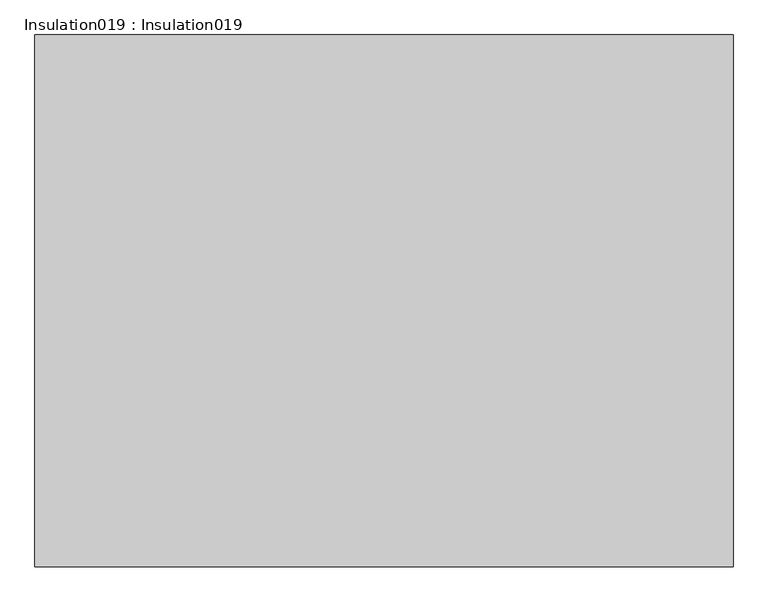
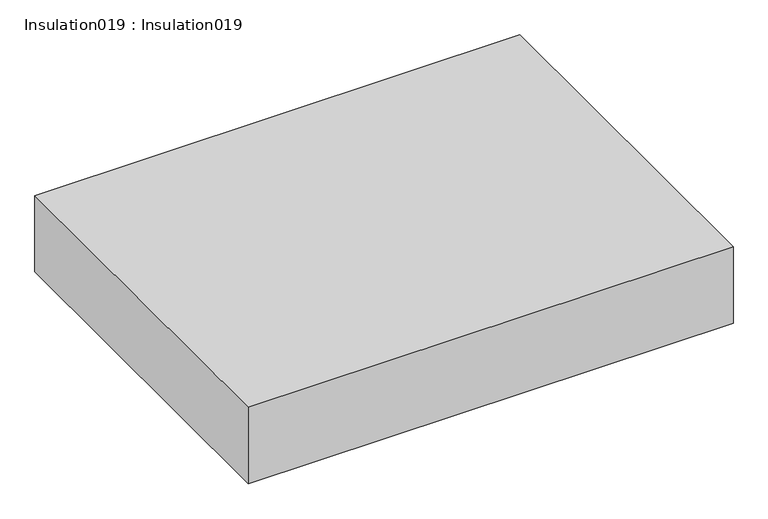
"""IFC4 building model written with IfcOpenShell, lengths in millimetres: proxy geometry, Insulation019 : Insulation019."""

import ifcopenshell
import ifcopenshell.guid

model = None  # the IFC model being written
_history = None  # IfcOwnerHistory: only IFC2X3 demands one
_inside = {}  # id of a spatial element -> (the spatial element, [elements in it])
_under = {}  # id of a project, library or spatial element -> (it, [spatial elements below it])
_declared = {}  # id of a project -> (the project, [libraries it declares])
_typed = {}  # id of a type object -> (the type object, [elements of that type])
_made_of = {}  # id of a material, layer set ... -> (it, [elements and type objects made of it])


def new_model(schema):
    """Start an empty IFC model of exactly this schema.

    Asked for "IFC4X3", IfcOpenShell would pick the latest addendum, in which some entities
    have other attributes; the version numbers below select the first issue.
    IFC2X3 requires an IfcOwnerHistory on every rooted entity: one is made here for all.
    """
    global model, _history
    if schema == "IFC4X3":
        model = ifcopenshell.file(schema_version=(4, 3, 0, 0))
    else:
        model = ifcopenshell.file(schema=schema)
    _inside.clear()
    _under.clear()
    _declared.clear()
    _typed.clear()
    _made_of.clear()
    _history = None
    if model.schema == "IFC2X3":
        org = make("IfcOrganization", Name="unknown")
        user = make(
            "IfcPersonAndOrganization",
            ThePerson=make("IfcPerson", FamilyName="unknown"),
            TheOrganization=org,
        )
        app = make(
            "IfcApplication",
            ApplicationDeveloper=org,
            Version="unknown",
            ApplicationFullName="unknown",
            ApplicationIdentifier="unknown",
        )
        _history = make(
            "IfcOwnerHistory",
            OwningUser=user,
            OwningApplication=app,
            ChangeAction="ADDED",
            CreationDate=0,
        )
    return model


def make(cls, **values):
    """One entity of the class cls with the attributes given. An attribute that is None is left unset."""
    return model.create_entity(
        cls, **{name: value for name, value in values.items() if value is not None}
    )


def rooted(cls, **values):
    """An entity with a GlobalId (a new one), such as an element, a storey or a relation."""
    return make(cls, GlobalId=ifcopenshell.guid.new(), OwnerHistory=_history, **values)


def si_unit(unit_type, name, prefix=None):
    """IfcSIUnit, for example si_unit("LENGTHUNIT", "METRE", prefix="MILLI")."""
    return make("IfcSIUnit", UnitType=unit_type, Prefix=prefix, Name=name)


def assignment(units):
    """IfcUnitAssignment: the units of a project."""
    return None if units is None else make("IfcUnitAssignment", Units=units)


def point(xyz):
    """IfcCartesianPoint."""
    return None if xyz is None else make("IfcCartesianPoint", Coordinates=xyz)


def direction(xyz):
    """IfcDirection."""
    return None if xyz is None else make("IfcDirection", DirectionRatios=xyz)


def frame(location, z_axis=None, x_axis=None):
    """IfcAxis2Placement3D, a coordinate frame: its origin and axes. An axis left out is left unset."""
    return make(
        "IfcAxis2Placement3D",
        Location=point(location),
        Axis=direction(z_axis),
        RefDirection=direction(x_axis),
    )


def origin():
    """The frame at (0, 0, 0) with its axes left unset."""
    return frame((0.0, 0.0, 0.0))


def place(relative_to, where):
    """IfcLocalPlacement: puts the frame where relative to a parent placement (None: the world)."""
    return make(
        "IfcLocalPlacement", PlacementRelTo=relative_to, RelativePlacement=where
    )


def context(
    kind, dimensions, precision=None, world=None, true_north=None, identifier=None
):
    """IfcGeometricRepresentationContext, for example the 3D "Model" context."""
    return make(
        "IfcGeometricRepresentationContext",
        ContextIdentifier=identifier,
        ContextType=kind,
        CoordinateSpaceDimension=dimensions,
        Precision=precision,
        WorldCoordinateSystem=world,
        TrueNorth=true_north,
    )


def project(units=None, contexts=None):
    """IfcProject with its units and contexts."""
    return rooted(
        "IfcProject",
        Name="project",
        RepresentationContexts=contexts,
        UnitsInContext=assignment(units),
    )


def spatial(cls, under=None, at=None, **own):
    """A site, building, storey or space (cls), placed at a placement, below another one or the project."""
    s = rooted(cls, ObjectPlacement=at, **own)
    if under is not None:
        _under.setdefault(under.id(), (under, []))[1].append(s)
    return s


def polyline(points):
    """IfcPolyline through the points."""
    return make("IfcPolyline", Points=[point(p) for p in points])


def outline(outer, holes=None, kind="AREA"):
    """IfcArbitraryClosedProfileDef: a profile drawn as a closed curve; with holes, ...WithVoids."""
    if holes is None:
        return make("IfcArbitraryClosedProfileDef", ProfileType=kind, OuterCurve=outer)
    return make(
        "IfcArbitraryProfileDefWithVoids",
        ProfileType=kind,
        OuterCurve=outer,
        InnerCurves=holes,
    )


def extrude(swept, where, along, depth):
    """IfcExtrudedAreaSolid: the profile swept, set in the frame where, extruded along a direction by depth."""
    return make(
        "IfcExtrudedAreaSolid",
        SweptArea=swept,
        Position=where,
        ExtrudedDirection=direction(along),
        Depth=depth,
    )


def shape(context_of_items, identifier, shape_type, items):
    """IfcShapeRepresentation: the items that make up one representation, for example the "Body"."""
    return make(
        "IfcShapeRepresentation",
        ContextOfItems=context_of_items,
        RepresentationIdentifier=identifier,
        RepresentationType=shape_type,
        Items=items,
    )


def source(mapping_origin, context_of_items, identifier, shape_type, items):
    """IfcRepresentationMap: a shape defined once, which mapped items show again and again."""
    return make(
        "IfcRepresentationMap",
        MappingOrigin=mapping_origin,
        MappedRepresentation=shape(context_of_items, identifier, shape_type, items),
    )


def transform(
    local_origin,
    x_axis=None,
    y_axis=None,
    z_axis=None,
    scale=None,
    scale2=None,
    scale3=None,
    uniform=True,
):
    """IfcCartesianTransformationOperator3D, or its non-uniform kind. x_axis, y_axis, z_axis: its Axis1, 2, 3."""
    if uniform:
        return make(
            "IfcCartesianTransformationOperator3D",
            Axis1=direction(x_axis),
            Axis2=direction(y_axis),
            LocalOrigin=point(local_origin),
            Scale=scale,
            Axis3=direction(z_axis),
        )
    return make(
        "IfcCartesianTransformationOperator3DnonUniform",
        Axis1=direction(x_axis),
        Axis2=direction(y_axis),
        LocalOrigin=point(local_origin),
        Scale=scale,
        Axis3=direction(z_axis),
        Scale2=scale2,
        Scale3=scale3,
    )


def mapped(mapping_source, mapping_target):
    """IfcMappedItem: shows the shape of a source again, moved by a transform."""
    return make(
        "IfcMappedItem", MappingSource=mapping_source, MappingTarget=mapping_target
    )


def made_of(thing, what):
    """Note that an element or type object is made of a material, layer set ...; save() writes the relation."""
    if what is not None:
        _made_of.setdefault(what.id(), (what, []))[1].append(thing)
    return thing


def element(
    cls,
    number,
    at=None,
    inside=None,
    cuts=None,
    type_object=None,
    material=None,
    context=None,
    identifier="Body",
    shape_type=None,
    held_by="IfcProductDefinitionShape",
    body=None,
    shapes=None,
    **own,
):
    """One element of the class cls, such as IfcWall. Its Tag is "e" and its number.

    at: its placement. inside: the storey or other place that contains it. cuts: it is an
    opening in that element (IfcRelVoidsElement). A single representation is given by context,
    identifier, shape_type and body (its items); several are given by shapes. held_by: the class
    of the entity that holds the representations. save() writes the other relations.
    """
    e = rooted(cls, Tag="e%d" % number, ObjectPlacement=at, **own)
    if body is not None:
        shapes = [shape(context, identifier, shape_type, body)]
    if shapes is not None:
        e.Representation = make(held_by, Representations=shapes)
    if inside is not None:
        _inside.setdefault(inside.id(), (inside, []))[1].append(e)
    if cuts is not None:
        rooted(
            "IfcRelVoidsElement", RelatingBuildingElement=cuts, RelatedOpeningElement=e
        )
    if type_object is not None:
        _typed.setdefault(type_object.id(), (type_object, []))[1].append(e)
    return made_of(e, material)


def aggregate(whole, parts):
    """IfcRelAggregates: a whole, such as a stair, and the parts it consists of."""
    return rooted("IfcRelAggregates", RelatingObject=whole, RelatedObjects=parts)


def save(model, path):
    """Write the relations noted so far, then the file.

    IfcRelAggregates (storeys below a building ...), IfcRelContainedInSpatialStructure (elements
    in a storey), IfcRelDefinesByType, IfcRelAssociatesMaterial and IfcRelDeclares: one each for
    every whole, place, type object, material and project.
    """
    for whole, parts in _under.values():
        aggregate(whole, parts)
    for where, things in _inside.values():
        rooted(
            "IfcRelContainedInSpatialStructure",
            RelatedElements=things,
            RelatingStructure=where,
        )
    for kind, things in _typed.values():
        rooted("IfcRelDefinesByType", RelatedObjects=things, RelatingType=kind)
    for what, things in _made_of.values():
        rooted("IfcRelAssociatesMaterial", RelatedObjects=things, RelatingMaterial=what)
    for by, libraries in _declared.values():
        rooted("IfcRelDeclares", RelatingContext=by, RelatedDefinitions=libraries)
    model.write(path)


def insulation019_insulation019_aaf8cb2f(model_context):
    return source(origin(), model_context, "Body", "SweptSolid", [
        extrude(outline(polyline([(12382.7678845, -4253.3675368), (12382.7678845, -2860.7425368), (14211.5678845, -2860.7425368), (14211.5678845, -4253.3675368), (12382.7678845, -4253.3675368)])), frame((0.0, 0.0, 39757.096), z_axis=(0.0, 0.0, 1.0), x_axis=(1.0, 0.0, 0.0)), (0.0, 0.0, 1.0), 304.8),
    ])


if __name__ == "__main__":
    model = new_model("IFC4")
    model_context = context("Model", 3, world=origin())
    ifc_project = project(units=[si_unit("LENGTHUNIT", "METRE", prefix="MILLI")], contexts=[model_context])
    site = spatial("IfcSite", under=ifc_project)
    building = spatial("IfcBuilding", under=site)
    placement = place(None, origin())
    insulation019_insulation019_shape = insulation019_insulation019_aaf8cb2f(model_context)
    element("IfcBuildingElementProxy", 1, Name="Insulation019 : Insulation019", ObjectType="Insulation019 : Insulation019", at=placement, inside=building, context=model_context, shape_type="MappedRepresentation", body=[
        mapped(insulation019_insulation019_shape, transform((0.0, 0.0, 0.0), x_axis=(1.0, 0.0, 0.0), y_axis=(0.0, 1.0, 0.0), z_axis=(0.0, 0.0, 1.0))),
    ])
    save(model, "model.ifc")

# Revit data of these elements
# Type "Insulation019 : Insulation019"
#   NameOverride = "Insulation019"
# Element 1 (IfcBuildingElementProxy, "Insulation019 : Insulation019")
#   Materials on its faces: "BATT INSULATION (U-FACTOR = 0.065 MIN.) OVER CLASS II VAPOR RETARDER (TOWARDS INTERIOR)"
# Materials
#   "BATT INSULATION (U-FACTOR = 0.065 MIN.) OVER CLASS II VAPOR RETARDER (TOWARDS INTERIOR)": class "Unassigned", colour RGB 246 242 160, transparency 0, Cost = 0
